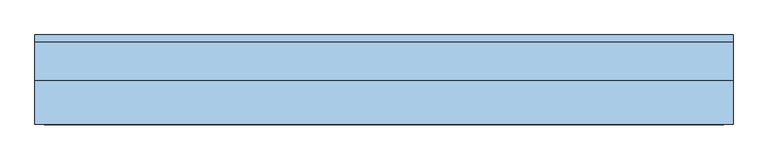
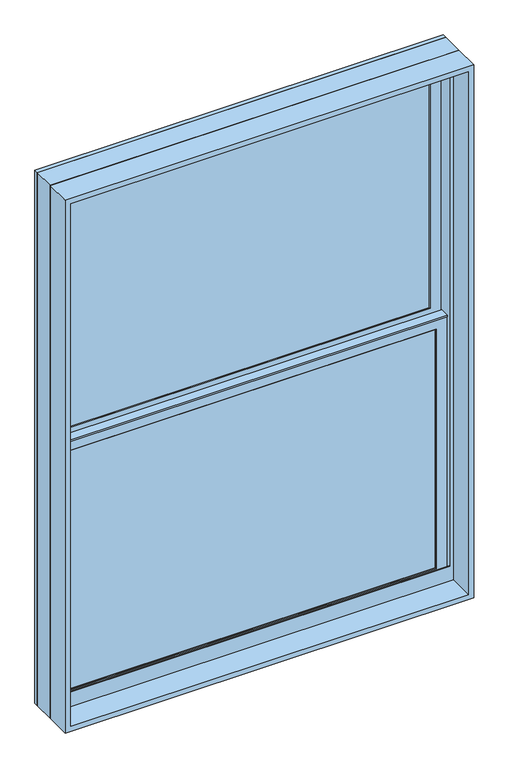
"""IFC4 building model written with IfcOpenShell, lengths in millimetres: window geometry, Window-Double_Hung-Marvin-Essential : ESDH4056."""

from ifc_helpers import new_model, si_unit, frame, origin, place, context, project, spatial, polyline, outline, extrude, faceted_brep, source, transform, mapped, element, save


def window_d1e83dd2(model_context):
    return source(origin(), model_context, "Body", "SolidModel", [
        extrude(outline(polyline([(191.5583333, 20.6375), (191.5583333, 15.875), (172.5083333, 15.875), (172.5083333, 20.6375), (191.5583333, 20.6375)])), frame((0.0, 0.0, 831.85), z_axis=(0.0, 0.0, 1.0), x_axis=(1.0, 0.0, 0.0)), (0.0, 0.0, 1.0), 755.65),
        extrude(outline(polyline([(-172.5083333, 20.6375), (-172.5083333, 15.875), (-191.5583333, 15.875), (-191.5583333, 20.6375), (-172.5083333, 20.6375)])), frame((0.0, 0.0, 831.85), z_axis=(0.0, 0.0, 1.0), x_axis=(1.0, 0.0, 0.0)), (0.0, 0.0, 1.0), 755.65),
        extrude(outline(polyline([(546.1, 20.6375), (546.1, 15.875), (-546.1, 15.875), (-546.1, 20.6375), (546.1, 20.6375)])), frame((0.0, 0.0, 1200.15), z_axis=(0.0, 0.0, 1.0), x_axis=(1.0, 0.0, 0.0)), (0.0, 0.0, 1.0), 19.05),
        extrude(outline(polyline([(-191.5583333, 46.83125), (-191.5583333, 51.59375), (-172.5083333, 51.59375), (-172.5083333, 46.83125), (-191.5583333, 46.83125)])), frame((0.0, 0.0, 1625.6), z_axis=(0.0, 0.0, 1.0), x_axis=(1.0, 0.0, 0.0)), (0.0, 0.0, 1.0), 755.65),
        extrude(outline(polyline([(172.5083333, 46.83125), (172.5083333, 51.59375), (191.5583333, 51.59375), (191.5583333, 46.83125), (172.5083333, 46.83125)])), frame((0.0, 0.0, 1625.6), z_axis=(0.0, 0.0, 1.0), x_axis=(1.0, 0.0, 0.0)), (0.0, 0.0, 1.0), 755.65),
        extrude(outline(polyline([(-546.1, 46.83125), (-546.1, 51.59375), (546.1, 51.59375), (546.1, 46.83125), (-546.1, 46.83125)])), frame((0.0, 0.0, 1993.9), z_axis=(0.0, 0.0, 1.0), x_axis=(1.0, 0.0, 0.0)), (0.0, 0.0, 1.0), 19.05),
        extrude(outline(polyline([(191.5583333, 20.6375), (172.5083333, 20.6375), (172.5083333, 25.4), (191.5583333, 25.4), (191.5583333, 20.6375)])), frame((0.0, 0.0, 831.85), z_axis=(0.0, 0.0, 1.0), x_axis=(1.0, 0.0, 0.0)), (0.0, 0.0, 1.0), 755.65),
        extrude(outline(polyline([(-172.5083333, 20.6375), (-191.5583333, 20.6375), (-191.5583333, 25.4), (-172.5083333, 25.4), (-172.5083333, 20.6375)])), frame((0.0, 0.0, 831.85), z_axis=(0.0, 0.0, 1.0), x_axis=(1.0, 0.0, 0.0)), (0.0, 0.0, 1.0), 755.65),
        extrude(outline(polyline([(546.1, 20.6375), (-546.1, 20.6375), (-546.1, 25.4), (546.1, 25.4), (546.1, 20.6375)])), frame((0.0, 0.0, 1200.15), z_axis=(0.0, 0.0, 1.0), x_axis=(1.0, 0.0, 0.0)), (0.0, 0.0, 1.0), 19.05),
        extrude(outline(polyline([(-191.5583333, 56.35625), (-172.5083333, 56.35625), (-172.5083333, 51.59375), (-191.5583333, 51.59375), (-191.5583333, 56.35625)])), frame((0.0, 0.0, 1625.6), z_axis=(0.0, 0.0, 1.0), x_axis=(1.0, 0.0, 0.0)), (0.0, 0.0, 1.0), 755.65),
        extrude(outline(polyline([(172.5083333, 56.35625), (191.5583333, 56.35625), (191.5583333, 51.59375), (172.5083333, 51.59375), (172.5083333, 56.35625)])), frame((0.0, 0.0, 1625.6), z_axis=(0.0, 0.0, 1.0), x_axis=(1.0, 0.0, 0.0)), (0.0, 0.0, 1.0), 755.65),
        extrude(outline(polyline([(-546.1, 56.35625), (546.1, 56.35625), (546.1, 51.59375), (-546.1, 51.59375), (-546.1, 56.35625)])), frame((0.0, 0.0, 1993.9), z_axis=(0.0, 0.0, 1.0), x_axis=(1.0, 0.0, 0.0)), (0.0, 0.0, 1.0), 19.05),
        faceted_brep([(-573.0875, 5.6780605, 1617.5351748), (-573.0875, 5.6780605, 1612.9), (573.0875, 5.6780605, 1612.9), (573.0875, 5.6780605, 1617.5351748), (-573.0875, 34.8118605, 1617.5351748), (573.0875, 34.8118605, 1617.5351748), (573.0875, 34.8118605, 1612.9), (-573.0875, 34.8118605, 1612.9), (-573.0875, 30.1625, 1612.9), (-573.0875, 30.1625, 804.8625), (-573.0875, 8.9241104, 804.8625), (-573.0875, 8.9241104, 1612.9), (573.0875, 8.9241104, 1612.9), (573.0875, 30.1625, 1612.9), (573.0875, 8.9241104, 804.8625), (573.0875, 30.1625, 804.8625), (-557.2034752, 11.90625, 1598.6034752), (-557.2034752, 30.1625, 1598.6034752), (557.2034752, 30.1625, 1598.6034752), (557.2034752, 11.90625, 1598.6034752), (-540.54375, 10.4662439, 1581.94375), (-540.54375, 11.90625, 1581.94375), (540.54375, 11.90625, 1581.94375), (540.54375, 10.4662439, 1581.94375), (542.0858834, 8.9241104, 1583.4858834), (-542.0858834, 8.9241104, 1583.4858834), (557.2034752, 30.1625, 820.7465248), (557.2034752, 11.90625, 820.7465248), (540.54375, 11.90625, 837.40625), (540.54375, 10.4662439, 837.40625), (542.0858834, 8.9241104, 835.8641166), (-557.2034752, 30.1625, 820.7465248), (-557.2034752, 11.90625, 820.7465248), (-540.54375, 11.90625, 837.40625), (-540.54375, 10.4662439, 837.40625), (-542.0858834, 8.9241104, 835.8641166)], [[[0, 1, 2, 3]], [[4, 5, 6, 7]], [[1, 0, 4, 7, 8, 9, 10, 11]], [[2, 1, 11, 12]], [[7, 6, 13, 8]], [[3, 2, 12, 14, 15, 13, 6, 5]], [[0, 3, 5, 4]], [[16, 17, 18, 19]], [[20, 21, 22, 23]], [[20, 23, 24, 25]], [[19, 18, 26, 27]], [[23, 22, 28, 29]], [[24, 23, 29, 30]], [[27, 26, 31, 32]], [[29, 28, 33, 34]], [[30, 29, 34, 35]], [[15, 14, 10, 9]], [[15, 9, 8, 13], [18, 17, 31, 26]], [[17, 16, 32, 31]], [[16, 19, 27, 32], [22, 21, 33, 28]], [[21, 20, 34, 33]], [[20, 25, 35, 34]], [[10, 14, 12, 11], [25, 24, 30, 35]]]),
        extrude(outline(polyline([(38.5955581, 1598.6125), (33.5778968, 1598.6125), (33.5778968, 1600.2), (39.9405976, 1600.2), (39.9405976, 1598.6125), (61.515625, 1598.6125), (47.6307501, 1595.2975159), (38.5955581, 1595.2975159), (38.5955581, 1598.6125)])), frame((-573.0875, 0.0, 0.0), z_axis=(1.0, 0.0, 0.0), x_axis=(0.0, 1.0, 0.0)), (0.0, 0.0, 1.0), 1146.175),
        faceted_brep([(603.25, 0.0, 774.7), (603.25, 0.0, 2438.4), (-603.25, 0.0, 2438.4), (-603.25, 0.0, 774.7), (577.05625, 0.0, 835.81875), (-577.05625, 0.0, 835.81875), (-577.05625, 0.0, 2412.20625), (577.05625, 0.0, 2412.20625), (577.05625, 3.96875, 774.7), (-577.05625, 3.96875, 774.7), (-577.05625, 3.96875, 835.81875), (577.05625, 3.96875, 835.81875), (-603.25, 65.6828125, 774.7), (-577.05625, 65.6828125, 774.7), (577.05625, 65.6828125, 774.7), (603.25, 65.6828125, 774.7), (-603.25, 65.6828125, 2438.4), (603.25, 65.6828125, 2438.4), (577.05625, 65.6828125, 2412.20625), (-577.05625, 65.6828125, 2412.20625)], [[[0, 1, 2, 3], [4, 5, 6, 7]], [[8, 9, 10, 11]], [[5, 4, 11, 10]], [[0, 3, 12, 13, 9, 8, 14, 15]], [[13, 12, 16, 17, 15, 14, 18, 19]], [[13, 19, 6, 5, 10, 9]], [[7, 6, 19, 18]], [[18, 14, 8, 11, 4, 7]], [[1, 0, 15, 17]], [[2, 1, 17, 16]], [[3, 2, 16, 12]]]),
        faceted_brep([(577.05625, 30.1625, 1606.55), (575.46875, 30.1625, 1606.55), (575.46875, 30.1625, 799.0544613), (577.05625, 30.1625, 799.0544613), (-575.46875, 30.1625, 1606.55), (-577.05625, 30.1625, 1606.55), (-577.05625, 30.1625, 799.0544613), (-575.46875, 30.1625, 799.0544613), (575.46875, 63.5, 1606.55), (577.05625, 63.5, 1606.55), (577.05625, 63.5, 792.5743077), (575.46875, 63.5, 792.5743077), (-577.05625, 63.5, 1606.55), (-575.46875, 63.5, 1606.55), (-575.46875, 63.5, 792.5743077), (-577.05625, 63.5, 792.5743077), (588.3108932, 3.96875, 804.1460105), (588.3108932, 3.96875, 774.7), (588.3108932, 65.6828125, 774.7), (588.3108932, 65.6828125, 792.150012), (-588.3108932, 3.96875, 774.7), (-588.3108932, 3.96875, 804.1460105), (-588.3108932, 65.6828125, 792.150012), (-588.3108932, 65.6828125, 774.7), (588.3108932, 78.58125, 789.6428097), (-588.3108932, 78.58125, 789.6428097), (-586.2971252, 68.2348864, 791.6539391), (-568.33135, 68.2348864, 791.6539391), (-568.33135, 65.6828125, 792.150012), (568.33135, 65.6828125, 792.150012), (568.33135, 68.2348864, 791.6539391), (586.2971252, 68.2348864, 791.6539391), (-603.25, 65.6828125, 774.7), (-603.25, 78.5948249, 774.7), (603.25, 78.5948249, 774.7), (603.25, 65.6828125, 774.7), (-603.25, 78.58125, 2438.4), (603.25, 78.58125, 2438.4), (588.3108932, 78.58125, 2423.4608932), (-588.3108932, 78.58125, 2423.4608932), (-603.25, 65.6828125, 2438.4), (-586.2971252, 68.2348864, 2421.4471252), (586.2971252, 68.2348864, 2421.4471252), (568.33135, 68.2348864, 2403.48135), (-568.33135, 68.2348864, 2403.48135), (-568.33135, 65.6828125, 2403.48135), (568.33135, 65.6828125, 2403.48135), (603.25, 65.6828125, 2438.4)], [[[0, 1, 2, 3]], [[4, 5, 6, 7]], [[8, 9, 10, 11]], [[12, 13, 14, 15]], [[1, 8, 11, 2]], [[9, 0, 3, 10]], [[1, 0, 9, 8]], [[5, 4, 13, 12]], [[5, 12, 15, 6]], [[13, 4, 7, 14]], [[16, 17, 18, 19]], [[20, 21, 22, 23]], [[24, 25, 26, 27, 28, 22, 21, 16, 19, 29, 30, 31], [3, 2, 11, 10], [7, 6, 15, 14]], [[17, 16, 21, 20]], [[17, 20, 23, 32, 33, 34, 35, 18]], [[34, 33, 36, 37], [25, 24, 38, 39]], [[33, 32, 40, 36]], [[39, 41, 26, 25]], [[41, 42, 31, 30, 43, 44, 27, 26]], [[44, 45, 28, 27]], [[40, 32, 23, 22, 28, 45, 46, 29, 19, 18, 35, 47]], [[36, 40, 47, 37]], [[39, 38, 42, 41]], [[44, 43, 46, 45]], [[34, 37, 47, 35]], [[42, 38, 24, 31]], [[46, 43, 30, 29]]]),
        extrude(outline(polyline([(553.24375, 11.90625), (-553.24375, 11.90625), (-553.24375, 15.08125), (553.24375, 15.08125), (553.24375, 11.90625)])), frame((0.0, 0.0, 824.70625), z_axis=(0.0, 0.0, 1.0), x_axis=(1.0, 0.0, 0.0)), (0.0, 0.0, 1.0), 769.9375),
        extrude(outline(polyline([(553.24375, 42.8625), (-553.24375, 42.8625), (-553.24375, 46.0375), (553.24375, 46.0375), (553.24375, 42.8625)])), frame((0.0, 0.0, 1618.45625), z_axis=(0.0, 0.0, 1.0), x_axis=(1.0, 0.0, 0.0)), (0.0, 0.0, 1.0), 769.9375),
        faceted_brep([(-540.54375, 31.194477, 1581.94375), (-542.0858834, 32.7366104, 1583.4858834), (542.0858834, 32.7366104, 1583.4858834), (540.54375, 31.194477, 1581.94375), (-540.54375, 30.1625, 1581.94375), (540.54375, 30.1625, 1581.94375), (-573.0875, 32.7366104, 1614.4875), (-573.0875, 30.1625, 1614.4875), (573.0875, 30.1625, 1614.4875), (573.0875, 32.7366104, 1614.4875), (542.0858834, 32.7366104, 835.8641166), (540.54375, 31.194477, 837.40625), (540.54375, 30.1625, 837.40625), (573.0875, 30.1625, 804.8625), (573.0875, 32.7366104, 804.8625), (-542.0858834, 32.7366104, 835.8641166), (-540.54375, 31.194477, 837.40625), (-540.54375, 30.1625, 837.40625), (-573.0875, 30.1625, 804.8625), (-573.0875, 32.7366104, 804.8625)], [[[0, 1, 2, 3]], [[4, 0, 3, 5]], [[6, 7, 8, 9]], [[3, 2, 10, 11]], [[5, 3, 11, 12]], [[9, 8, 13, 14]], [[11, 10, 15, 16]], [[12, 11, 16, 17]], [[14, 13, 18, 19]], [[9, 14, 19, 6], [1, 15, 10, 2]], [[16, 15, 1, 0]], [[17, 16, 0, 4]], [[7, 18, 13, 8], [5, 12, 17, 4]], [[19, 18, 7, 6]]]),
        faceted_brep([(-557.2034752, 42.8625, 2392.3534752), (-557.2034752, 61.11875, 2392.3534752), (557.2034752, 61.11875, 2392.3534752), (557.2034752, 42.8625, 2392.3534752), (-540.54375, 41.4224939, 2375.69375), (-540.54375, 42.8625, 2375.69375), (540.54375, 42.8625, 2375.69375), (540.54375, 41.4224939, 2375.69375), (-542.0858834, 39.8803604, 2377.2358834), (542.0858834, 39.8803604, 2377.2358834), (-573.0875, 61.11875, 2408.2375), (-573.0875, 39.8803604, 2408.2375), (573.0875, 39.8803604, 2408.2375), (573.0875, 61.11875, 2408.2375), (557.2034752, 61.11875, 1614.4965248), (557.2034752, 42.8625, 1614.4965248), (540.54375, 42.8625, 1631.15625), (540.54375, 41.4224939, 1631.15625), (542.0858834, 39.8803604, 1629.6141166), (573.0875, 39.8803604, 1598.6125), (573.0875, 61.11875, 1598.6125), (-557.2034752, 61.11875, 1614.4965248), (-557.2034752, 42.8625, 1614.4965248), (-540.54375, 42.8625, 1631.15625), (-540.54375, 41.4224939, 1631.15625), (-542.0858834, 39.8803604, 1629.6141166), (-573.0875, 39.8803604, 1598.6125), (-573.0875, 61.11875, 1598.6125)], [[[0, 1, 2, 3]], [[4, 5, 6, 7]], [[8, 4, 7, 9]], [[10, 11, 12, 13]], [[3, 2, 14, 15]], [[7, 6, 16, 17]], [[9, 7, 17, 18]], [[13, 12, 19, 20]], [[15, 14, 21, 22]], [[17, 16, 23, 24]], [[18, 17, 24, 25]], [[20, 19, 26, 27]], [[13, 20, 27, 10], [1, 21, 14, 2]], [[22, 21, 1, 0]], [[3, 15, 22, 0], [5, 23, 16, 6]], [[24, 23, 5, 4]], [[25, 24, 4, 8]], [[11, 26, 19, 12], [9, 18, 25, 8]], [[27, 26, 11, 10]]]),
        faceted_brep([(-573.0875, 61.11875, 1598.6125), (-573.0875, 63.6928604, 1598.6125), (573.0875, 63.6928604, 1598.6125), (573.0875, 61.11875, 1598.6125), (-540.54375, 62.150727, 1631.15625), (-540.54375, 61.11875, 1631.15625), (540.54375, 61.11875, 1631.15625), (540.54375, 62.150727, 1631.15625), (-542.0858834, 63.6928604, 1629.6141166), (542.0858834, 63.6928604, 1629.6141166), (573.0875, 63.6928604, 2408.2375), (573.0875, 61.11875, 2408.2375), (540.54375, 61.11875, 2375.69375), (540.54375, 62.150727, 2375.69375), (542.0858834, 63.6928604, 2377.2358834), (-573.0875, 63.6928604, 2408.2375), (-573.0875, 61.11875, 2408.2375), (-540.54375, 61.11875, 2375.69375), (-540.54375, 62.150727, 2375.69375), (-542.0858834, 63.6928604, 2377.2358834)], [[[0, 1, 2, 3]], [[4, 5, 6, 7]], [[8, 4, 7, 9]], [[3, 2, 10, 11]], [[7, 6, 12, 13]], [[9, 7, 13, 14]], [[11, 10, 15, 16]], [[13, 12, 17, 18]], [[14, 13, 18, 19]], [[16, 15, 1, 0]], [[3, 11, 16, 0], [5, 17, 12, 6]], [[18, 17, 5, 4]], [[19, 18, 4, 8]], [[1, 15, 10, 2], [9, 14, 19, 8]]]),
        extrude(outline(polyline([(553.24375, 26.19375), (-553.24375, 26.19375), (-553.24375, 30.1625), (553.24375, 30.1625), (553.24375, 26.19375)])), frame((0.0, 0.0, 824.70625), z_axis=(0.0, 0.0, 1.0), x_axis=(1.0, 0.0, 0.0)), (0.0, 0.0, 1.0), 769.9375),
        extrude(outline(polyline([(553.24375, 57.15), (-553.24375, 57.15), (-553.24375, 61.11875), (553.24375, 61.11875), (553.24375, 57.15)])), frame((0.0, 0.0, 1618.45625), z_axis=(0.0, 0.0, 1.0), x_axis=(1.0, 0.0, 0.0)), (0.0, 0.0, 1.0), 769.9375),
        extrude(outline(polyline([(2438.4, 603.25), (2438.4, -603.25), (774.7, -603.25), (774.7, 603.25), (2438.4, 603.25)]), holes=[polyline([(2422.525, 587.375), (790.575, 587.375), (790.575, -587.375), (2422.525, -587.375), (2422.525, 587.375)])]), frame((0.0, -76.2, 0.0), z_axis=(0.0, 1.0, 0.0), x_axis=(0.0, 0.0, 1.0)), (0.0, 0.0, 1.0), 75.40625),
    ])


if __name__ == "__main__":
    model = new_model("IFC4")
    model_context = context("Model", 3, world=origin())
    ifc_project = project(units=[si_unit("LENGTHUNIT", "METRE", prefix="MILLI")], contexts=[model_context])
    site = spatial("IfcSite", under=ifc_project)
    building = spatial("IfcBuilding", under=site)
    placement = place(None, origin())
    window_shape = window_d1e83dd2(model_context)
    element("IfcWindow", 1, ObjectType="Window-Double_Hung-Marvin-Essential : ESDH4056", at=placement, inside=building, context=model_context, shape_type="MappedRepresentation", body=[
        mapped(window_shape, transform((0.0, 0.0, 0.0), x_axis=(1.0, 0.0, 0.0), y_axis=(0.0, 1.0, 0.0), z_axis=(0.0, 0.0, 1.0))),
    ])
    save(model, "model.ifc")

# Revit data of these elements
# Type "Window-Double_Hung-Marvin-Essential : ESDH4056"
#   Type Mark = "74"
#   Window Type = "Essential Double Hung"
#   Product data url = "https://bimobject.com/marvin-windows-and-doors/product/marvin-dhwau"
#   Product Guid = "c4a96547-874c-4385-91dc-a058adc19d98"
#   Frame = "All Ultrex"
#   Egress Window = "Yes"
#   URL = "www.marvin.com"
#   Model = "ESDH4056"
#   Manufacturer = "Marvin Windows and Doors"
#   Label Egress = "EGRESS WDW"
#   Glass Type = "IG Low E II with Argon"
#   Design Pressure = "DP30"
#   Description = "4866 DBHG"
#   Analytic Construction = "<None>"
#   Prairie Corner Width = 0' - 4"
#   Prairie Corner Height = 0' - 4"
#   Egress Width = 3' - 8 9/16"
#   Egress Height = 2' - 4 27/128"
#   Rough Width = 4' - 0"
#   Rough Height = 5' - 6"
#   Nominal Width = 4' - 0"
#   Nominal Height = 5' - 6"
#   Inset to Installation Flange [instance default] = 0' - 1"
#   Height = 5' - 5 1/2"
#   Egress Area = 8.73021 SF
#   Default Head Height = 8' - 0"
#   Width = 3' - 11 1/2"
#   Daylight Area = 17.328 SF
#   DLO Width = 3' - 6 9/16"
#   DLO Height = 2' - 5 5/16"
#   Muntins Top Sash = yes
#   Lites Wide Top Sash = 3
#   Lites Wide Bottom Sash = 3
#   Lites High Top Sash = 2
#   Lites High Bottom Sash = 2
#   Lite Cut Prairie 9 = no
#   Lite Cut HV Grid = yes
#   Muntins Bottom Sash = yes
#   Label Visibility = no
#   Jamb Extension Visibility = yes
#   Edition number = 1
#   Interior Material = Ultrex-Marvin-Stonewhite
#   Glazing Material = Glass-Marvin-IG Low E II with Argon
#   Cladding Material = Ultrex-Marvin-Pebblegray
#   Wall Closure = (empty or 0)
#   Assembly Code = ""
# Element 1 (IfcWindow, "Window-Double_Hung-Marvin-Essential : ESDH4056")
#   Materials on its faces: "Ultrex-Marvin-Pebblegray", "Ultrex-Marvin-Stonewhite", "Glass-Marvin-IG Low E II with Argon"
# Materials
#   "Ultrex-Marvin-Stonewhite": class "Paint", colour RGB 250 251 245, transparency 0
#   "Glass-Marvin-IG Low E II with Argon": class "Glass", colour RGB 0 128 192, transparency 0.85
#   "Ultrex-Marvin-Pebblegray": class "Paint", colour RGB 189 185 173, transparency 0
